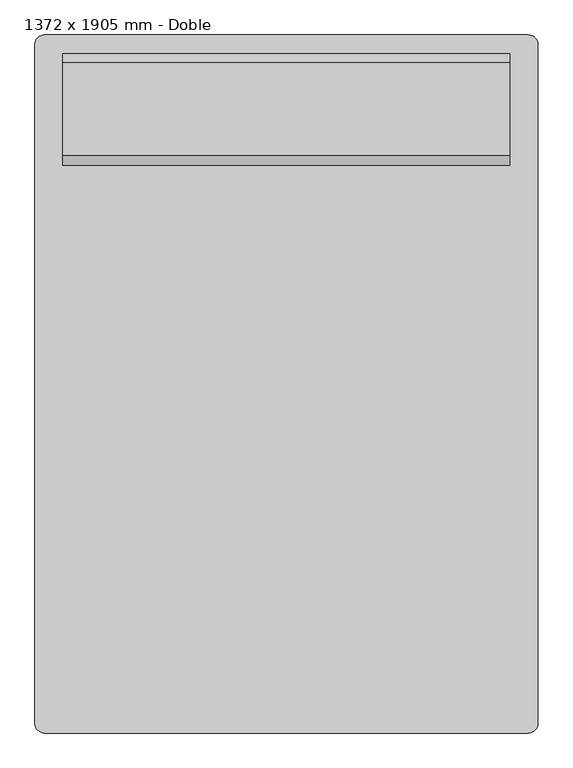
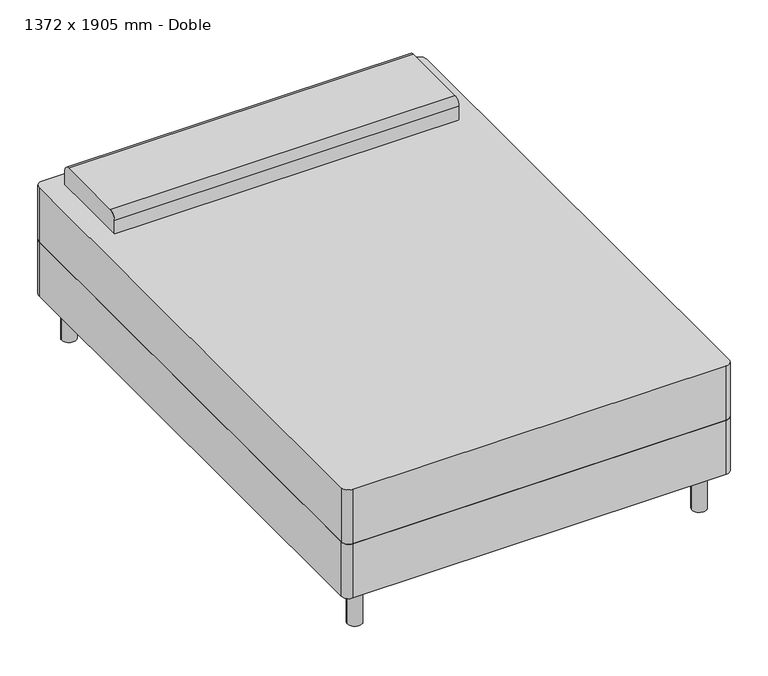
"""IFC4 building model written with IfcOpenShell, lengths in millimetres: furniture geometry, Cama-Estándar : 1372 x 1905 mm - Doble."""

import ifcopenshell
import ifcopenshell.guid

model = None  # the IFC model being written
_history = None  # IfcOwnerHistory: only IFC2X3 demands one
_inside = {}  # id of a spatial element -> (the spatial element, [elements in it])
_under = {}  # id of a project, library or spatial element -> (it, [spatial elements below it])
_declared = {}  # id of a project -> (the project, [libraries it declares])
_typed = {}  # id of a type object -> (the type object, [elements of that type])
_made_of = {}  # id of a material, layer set ... -> (it, [elements and type objects made of it])


def new_model(schema):
    """Start an empty IFC model of exactly this schema.

    Asked for "IFC4X3", IfcOpenShell would pick the latest addendum, in which some entities
    have other attributes; the version numbers below select the first issue.
    IFC2X3 requires an IfcOwnerHistory on every rooted entity: one is made here for all.
    """
    global model, _history
    if schema == "IFC4X3":
        model = ifcopenshell.file(schema_version=(4, 3, 0, 0))
    else:
        model = ifcopenshell.file(schema=schema)
    _inside.clear()
    _under.clear()
    _declared.clear()
    _typed.clear()
    _made_of.clear()
    _history = None
    if model.schema == "IFC2X3":
        org = make("IfcOrganization", Name="unknown")
        user = make(
            "IfcPersonAndOrganization",
            ThePerson=make("IfcPerson", FamilyName="unknown"),
            TheOrganization=org,
        )
        app = make(
            "IfcApplication",
            ApplicationDeveloper=org,
            Version="unknown",
            ApplicationFullName="unknown",
            ApplicationIdentifier="unknown",
        )
        _history = make(
            "IfcOwnerHistory",
            OwningUser=user,
            OwningApplication=app,
            ChangeAction="ADDED",
            CreationDate=0,
        )
    return model


def make(cls, **values):
    """One entity of the class cls with the attributes given. An attribute that is None is left unset."""
    return model.create_entity(
        cls, **{name: value for name, value in values.items() if value is not None}
    )


def rooted(cls, **values):
    """An entity with a GlobalId (a new one), such as an element, a storey or a relation."""
    return make(cls, GlobalId=ifcopenshell.guid.new(), OwnerHistory=_history, **values)


def si_unit(unit_type, name, prefix=None):
    """IfcSIUnit, for example si_unit("LENGTHUNIT", "METRE", prefix="MILLI")."""
    return make("IfcSIUnit", UnitType=unit_type, Prefix=prefix, Name=name)


def assignment(units):
    """IfcUnitAssignment: the units of a project."""
    return None if units is None else make("IfcUnitAssignment", Units=units)


def point(xyz):
    """IfcCartesianPoint."""
    return None if xyz is None else make("IfcCartesianPoint", Coordinates=xyz)


def direction(xyz):
    """IfcDirection."""
    return None if xyz is None else make("IfcDirection", DirectionRatios=xyz)


def frame(location, z_axis=None, x_axis=None):
    """IfcAxis2Placement3D, a coordinate frame: its origin and axes. An axis left out is left unset."""
    return make(
        "IfcAxis2Placement3D",
        Location=point(location),
        Axis=direction(z_axis),
        RefDirection=direction(x_axis),
    )


def frame_2d(location, x_axis=None):
    """IfcAxis2Placement2D, a coordinate frame in the plane: its origin and x axis."""
    return make(
        "IfcAxis2Placement2D", Location=point(location), RefDirection=direction(x_axis)
    )


def origin():
    """The frame at (0, 0, 0) with its axes left unset."""
    return frame((0.0, 0.0, 0.0))


def origin_with_axes():
    """The frame at (0, 0, 0) with the z axis (0, 0, 1) and the x axis (1, 0, 0) written out."""
    return frame((0.0, 0.0, 0.0), z_axis=(0.0, 0.0, 1.0), x_axis=(1.0, 0.0, 0.0))


def place(relative_to, where):
    """IfcLocalPlacement: puts the frame where relative to a parent placement (None: the world)."""
    return make(
        "IfcLocalPlacement", PlacementRelTo=relative_to, RelativePlacement=where
    )


def context(
    kind, dimensions, precision=None, world=None, true_north=None, identifier=None
):
    """IfcGeometricRepresentationContext, for example the 3D "Model" context."""
    return make(
        "IfcGeometricRepresentationContext",
        ContextIdentifier=identifier,
        ContextType=kind,
        CoordinateSpaceDimension=dimensions,
        Precision=precision,
        WorldCoordinateSystem=world,
        TrueNorth=true_north,
    )


def project(units=None, contexts=None):
    """IfcProject with its units and contexts."""
    return rooted(
        "IfcProject",
        Name="project",
        RepresentationContexts=contexts,
        UnitsInContext=assignment(units),
    )


def spatial(cls, under=None, at=None, **own):
    """A site, building, storey or space (cls), placed at a placement, below another one or the project."""
    s = rooted(cls, ObjectPlacement=at, **own)
    if under is not None:
        _under.setdefault(under.id(), (under, []))[1].append(s)
    return s


def polyline(points):
    """IfcPolyline through the points."""
    return make("IfcPolyline", Points=[point(p) for p in points])


def circle_curve(where, radius):
    """IfcCircle in the frame where."""
    return make("IfcCircle", Position=where, Radius=radius)


def trimmed(basis, trim1, trim2, sense, master):
    """IfcTrimmedCurve: the piece of a basis curve between two trims."""
    return make(
        "IfcTrimmedCurve",
        BasisCurve=basis,
        Trim1=trim1,
        Trim2=trim2,
        SenseAgreement=sense,
        MasterRepresentation=master,
    )


def segment(curve, same_sense, transition):
    """IfcCompositeCurveSegment."""
    return make(
        "IfcCompositeCurveSegment",
        Transition=transition,
        SameSense=same_sense,
        ParentCurve=curve,
    )


def composite_curve(segments, self_intersect=None):
    """IfcCompositeCurve: segments joined end to end."""
    return make("IfcCompositeCurve", Segments=segments, SelfIntersect=self_intersect)


def outline(outer, holes=None, kind="AREA"):
    """IfcArbitraryClosedProfileDef: a profile drawn as a closed curve; with holes, ...WithVoids."""
    if holes is None:
        return make("IfcArbitraryClosedProfileDef", ProfileType=kind, OuterCurve=outer)
    return make(
        "IfcArbitraryProfileDefWithVoids",
        ProfileType=kind,
        OuterCurve=outer,
        InnerCurves=holes,
    )


def extrude(swept, where, along, depth):
    """IfcExtrudedAreaSolid: the profile swept, set in the frame where, extruded along a direction by depth."""
    return make(
        "IfcExtrudedAreaSolid",
        SweptArea=swept,
        Position=where,
        ExtrudedDirection=direction(along),
        Depth=depth,
    )


def shape(context_of_items, identifier, shape_type, items):
    """IfcShapeRepresentation: the items that make up one representation, for example the "Body"."""
    return make(
        "IfcShapeRepresentation",
        ContextOfItems=context_of_items,
        RepresentationIdentifier=identifier,
        RepresentationType=shape_type,
        Items=items,
    )


def source(mapping_origin, context_of_items, identifier, shape_type, items):
    """IfcRepresentationMap: a shape defined once, which mapped items show again and again."""
    return make(
        "IfcRepresentationMap",
        MappingOrigin=mapping_origin,
        MappedRepresentation=shape(context_of_items, identifier, shape_type, items),
    )


def transform(
    local_origin,
    x_axis=None,
    y_axis=None,
    z_axis=None,
    scale=None,
    scale2=None,
    scale3=None,
    uniform=True,
):
    """IfcCartesianTransformationOperator3D, or its non-uniform kind. x_axis, y_axis, z_axis: its Axis1, 2, 3."""
    if uniform:
        return make(
            "IfcCartesianTransformationOperator3D",
            Axis1=direction(x_axis),
            Axis2=direction(y_axis),
            LocalOrigin=point(local_origin),
            Scale=scale,
            Axis3=direction(z_axis),
        )
    return make(
        "IfcCartesianTransformationOperator3DnonUniform",
        Axis1=direction(x_axis),
        Axis2=direction(y_axis),
        LocalOrigin=point(local_origin),
        Scale=scale,
        Axis3=direction(z_axis),
        Scale2=scale2,
        Scale3=scale3,
    )


def mapped(mapping_source, mapping_target):
    """IfcMappedItem: shows the shape of a source again, moved by a transform."""
    return make(
        "IfcMappedItem", MappingSource=mapping_source, MappingTarget=mapping_target
    )


def made_of(thing, what):
    """Note that an element or type object is made of a material, layer set ...; save() writes the relation."""
    if what is not None:
        _made_of.setdefault(what.id(), (what, []))[1].append(thing)
    return thing


def element(
    cls,
    number,
    at=None,
    inside=None,
    cuts=None,
    type_object=None,
    material=None,
    context=None,
    identifier="Body",
    shape_type=None,
    held_by="IfcProductDefinitionShape",
    body=None,
    shapes=None,
    **own,
):
    """One element of the class cls, such as IfcWall. Its Tag is "e" and its number.

    at: its placement. inside: the storey or other place that contains it. cuts: it is an
    opening in that element (IfcRelVoidsElement). A single representation is given by context,
    identifier, shape_type and body (its items); several are given by shapes. held_by: the class
    of the entity that holds the representations. save() writes the other relations.
    """
    e = rooted(cls, Tag="e%d" % number, ObjectPlacement=at, **own)
    if body is not None:
        shapes = [shape(context, identifier, shape_type, body)]
    if shapes is not None:
        e.Representation = make(held_by, Representations=shapes)
    if inside is not None:
        _inside.setdefault(inside.id(), (inside, []))[1].append(e)
    if cuts is not None:
        rooted(
            "IfcRelVoidsElement", RelatingBuildingElement=cuts, RelatedOpeningElement=e
        )
    if type_object is not None:
        _typed.setdefault(type_object.id(), (type_object, []))[1].append(e)
    return made_of(e, material)


def aggregate(whole, parts):
    """IfcRelAggregates: a whole, such as a stair, and the parts it consists of."""
    return rooted("IfcRelAggregates", RelatingObject=whole, RelatedObjects=parts)


def save(model, path):
    """Write the relations noted so far, then the file.

    IfcRelAggregates (storeys below a building ...), IfcRelContainedInSpatialStructure (elements
    in a storey), IfcRelDefinesByType, IfcRelAssociatesMaterial and IfcRelDeclares: one each for
    every whole, place, type object, material and project.
    """
    for whole, parts in _under.values():
        aggregate(whole, parts)
    for where, things in _inside.values():
        rooted(
            "IfcRelContainedInSpatialStructure",
            RelatedElements=things,
            RelatingStructure=where,
        )
    for kind, things in _typed.values():
        rooted("IfcRelDefinesByType", RelatedObjects=things, RelatingType=kind)
    for what, things in _made_of.values():
        rooted("IfcRelAssociatesMaterial", RelatedObjects=things, RelatingMaterial=what)
    for by, libraries in _declared.values():
        rooted("IfcRelDeclares", RelatingContext=by, RelatedDefinitions=libraries)
    model.write(path)


def furniture_1372_x_1905_mm_doble_2dcc4a2e(model_context):
    return source(origin(), model_context, "Body", "SweptSolid", [
        extrude(outline(composite_curve([segment(polyline([(-414.5114754, -972.695082), (-414.5114754, 881.504918)]), True, "CONTINUOUS"), segment(trimmed(circle_curve(frame_2d((-389.1114754, 881.504918)), 25.4), [point((-414.5114754, 881.504918))], [point((-389.1114754, 906.904918))], False, "CARTESIAN"), True, "CONTINUOUS"), segment(polyline([(-389.1114754, 906.904918), (932.0885246, 906.904918)]), True, "CONTINUOUS"), segment(trimmed(circle_curve(frame_2d((932.0885246, 881.504918)), 25.4), [point((932.0885246, 906.904918))], [point((957.4885246, 881.504918))], False, "CARTESIAN"), True, "CONTINUOUS"), segment(polyline([(957.4885246, 881.504918), (957.4885246, -972.695082)]), True, "CONTINUOUS"), segment(trimmed(circle_curve(frame_2d((932.0885246, -972.695082)), 25.4), [point((957.4885246, -972.695082))], [point((932.0885246, -998.095082))], False, "CARTESIAN"), True, "CONTINUOUS"), segment(polyline([(932.0885246, -998.095082), (-389.1114754, -998.095082)]), True, "CONTINUOUS"), segment(trimmed(circle_curve(frame_2d((-389.1114754, -972.695082)), 25.4), [point((-389.1114754, -998.095082))], [point((-414.5114754, -972.695082))], False, "CARTESIAN"), True, "CONTINUOUS")], self_intersect=False)), frame((0.0, 0.0, 152.4), z_axis=(0.0, 0.0, 1.0), x_axis=(1.0, 0.0, 0.0)), (0.0, 0.0, 1.0), 203.2),
        extrude(outline(composite_curve([segment(polyline([(551.304918, 558.8), (551.304918, 609.6)]), True, "CONTINUOUS"), segment(trimmed(circle_curve(frame_2d((576.704918, 609.6)), 25.4), [point((551.304918, 609.6))], [point((576.704918, 635.0))], False, "CARTESIAN"), True, "CONTINUOUS"), segment(polyline([(576.704918, 635.0), (830.704918, 635.0)]), True, "CONTINUOUS"), segment(trimmed(circle_curve(frame_2d((830.704918, 609.6)), 25.4), [point((830.704918, 635.0))], [point((856.104918, 609.6))], False, "CARTESIAN"), True, "CONTINUOUS"), segment(polyline([(856.104918, 609.6), (856.104918, 558.8), (551.304918, 558.8)]), True, "CONTINUOUS")], self_intersect=False)), frame((-338.3114754, 0.0, 0.0), z_axis=(1.0, 0.0, 0.0), x_axis=(0.0, 1.0, 0.0)), (0.0, 0.0, 1.0), 1219.6),
        extrude(outline(composite_curve([segment(trimmed(circle_curve(frame_2d((-338.3114754, 830.704918)), 25.4), [point((-363.7114754, 830.704918))], [point((-312.9114754, 830.704918))], False, "CARTESIAN"), True, "CONTINUOUS"), segment(trimmed(circle_curve(frame_2d((-338.3114754, 830.704918)), 25.4), [point((-312.9114754, 830.704918))], [point((-363.7114754, 830.704918))], False, "CARTESIAN"), True, "CONTINUOUS")], self_intersect=False)), origin_with_axes(), (0.0, 0.0, 1.0), 152.4),
        extrude(outline(composite_curve([segment(trimmed(circle_curve(frame_2d((881.2885246, 830.704918)), 25.4), [point((855.8885246, 830.704918))], [point((906.6885246, 830.704918))], False, "CARTESIAN"), True, "CONTINUOUS"), segment(trimmed(circle_curve(frame_2d((881.2885246, 830.704918)), 25.4), [point((906.6885246, 830.704918))], [point((855.8885246, 830.704918))], False, "CARTESIAN"), True, "CONTINUOUS")], self_intersect=False)), origin_with_axes(), (0.0, 0.0, 1.0), 152.4),
        extrude(outline(composite_curve([segment(trimmed(circle_curve(frame_2d((881.2885246, -921.895082)), 25.4), [point((855.8885246, -921.895082))], [point((906.6885246, -921.895082))], False, "CARTESIAN"), True, "CONTINUOUS"), segment(trimmed(circle_curve(frame_2d((881.2885246, -921.895082)), 25.4), [point((906.6885246, -921.895082))], [point((855.8885246, -921.895082))], False, "CARTESIAN"), True, "CONTINUOUS")], self_intersect=False)), origin_with_axes(), (0.0, 0.0, 1.0), 152.4),
        extrude(outline(composite_curve([segment(trimmed(circle_curve(frame_2d((-338.3114754, -921.895082)), 25.4), [point((-363.7114754, -921.895082))], [point((-312.9114754, -921.895082))], False, "CARTESIAN"), True, "CONTINUOUS"), segment(trimmed(circle_curve(frame_2d((-338.3114754, -921.895082)), 25.4), [point((-312.9114754, -921.895082))], [point((-363.7114754, -921.895082))], False, "CARTESIAN"), True, "CONTINUOUS")], self_intersect=False)), origin_with_axes(), (0.0, 0.0, 1.0), 152.4),
        extrude(outline(composite_curve([segment(polyline([(-389.1114754, 906.904918), (932.0885246, 906.904918)]), True, "CONTINUOUS"), segment(trimmed(circle_curve(frame_2d((932.0885246, 881.504918)), 25.4), [point((932.0885246, 906.904918))], [point((957.4885246, 881.504918))], False, "CARTESIAN"), True, "CONTINUOUS"), segment(polyline([(957.4885246, 881.504918), (957.4885246, -972.695082)]), True, "CONTINUOUS"), segment(trimmed(circle_curve(frame_2d((932.0885246, -972.695082)), 25.4), [point((957.4885246, -972.695082))], [point((932.0885246, -998.095082))], False, "CARTESIAN"), True, "CONTINUOUS"), segment(polyline([(932.0885246, -998.095082), (-389.1114754, -998.095082)]), True, "CONTINUOUS"), segment(trimmed(circle_curve(frame_2d((-389.1114754, -972.695082)), 25.4), [point((-389.1114754, -998.095082))], [point((-414.5114754, -972.695082))], False, "CARTESIAN"), True, "CONTINUOUS"), segment(polyline([(-414.5114754, -972.695082), (-414.5114754, 881.504918)]), True, "CONTINUOUS"), segment(trimmed(circle_curve(frame_2d((-389.1114754, 881.504918)), 25.4), [point((-414.5114754, 881.504918))], [point((-389.1114754, 906.904918))], False, "CARTESIAN"), True, "CONTINUOUS")], self_intersect=False)), frame((0.0, 0.0, 355.6), z_axis=(0.0, 0.0, 1.0), x_axis=(1.0, 0.0, 0.0)), (0.0, 0.0, 1.0), 203.2),
    ])


if __name__ == "__main__":
    model = new_model("IFC4")
    model_context = context("Model", 3, world=origin())
    ifc_project = project(units=[si_unit("LENGTHUNIT", "METRE", prefix="MILLI")], contexts=[model_context])
    site = spatial("IfcSite", under=ifc_project)
    building = spatial("IfcBuilding", under=site)
    placement = place(None, origin())
    furniture_1372_x_1905_mm_doble_shape = furniture_1372_x_1905_mm_doble_2dcc4a2e(model_context)
    element("IfcFurniture", 1, ObjectType="Cama-Estándar : 1372 x 1905 mm - Doble", at=placement, inside=building, context=model_context, shape_type="MappedRepresentation", body=[
        mapped(furniture_1372_x_1905_mm_doble_shape, transform((0.0, 0.0, 0.0), x_axis=(1.0, 0.0, 0.0), y_axis=(0.0, 1.0, 0.0), z_axis=(0.0, 0.0, 1.0))),
    ])
    save(model, "model.ifc")

# Revit data of these elements
# Type "Cama-Estándar : 1372 x 1905 mm - Doble"
#   Longitud = 1.905 m
#   Anchura = 1.372 m
#   Máscara [instance default] = yes
#   Material de soporte = Metal - Cromo
#   Material de colchón = Textil - Blanco
#   Default Elevation = 0
# Element 1 (IfcFurniture, "Cama-Estándar : 1372 x 1905 mm - Doble")
#   Materials on its faces: "Metal - Cromo", "Textil - Blanco"
# Materials
#   "Metal - Cromo": class "Metal", colour RGB 17 17 17, transparency 0
#   "Textil - Blanco": class "Tela", colour RGB 247 247 239, transparency 0
